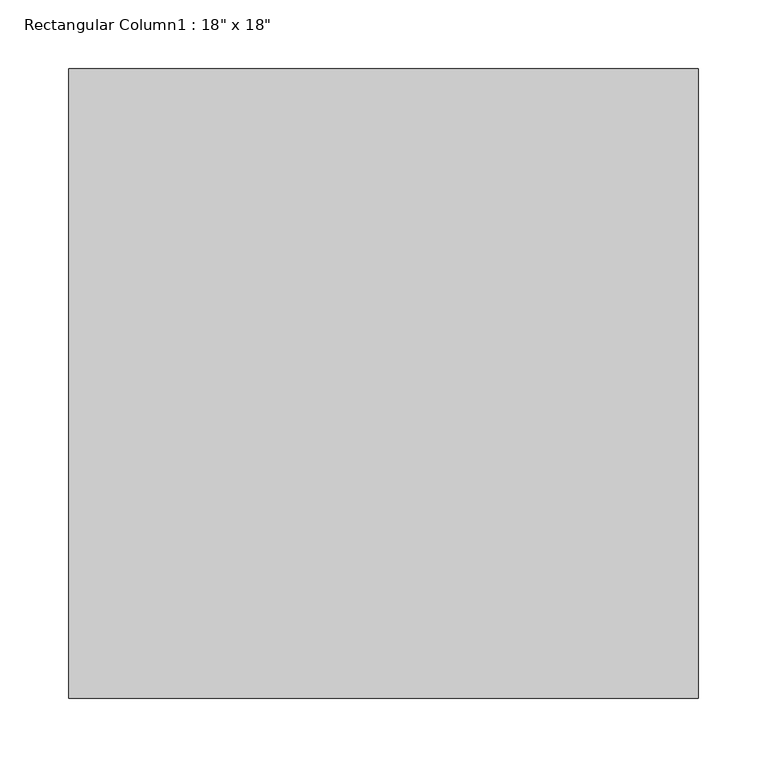
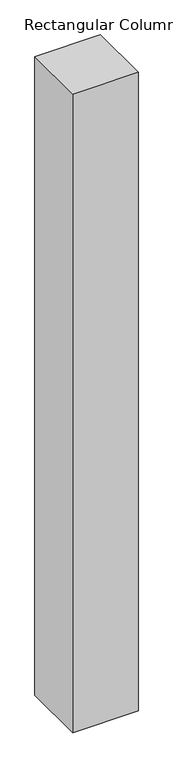
"""IFC4 building model written with IfcOpenShell, lengths in millimetres: column geometry."""

from ifc_helpers import new_model, si_unit, frame, origin, place, context, project, spatial, polyline, outline, extrude, source, transform, mapped, element, save


def column_773d994b(model_context):
    return source(origin(), model_context, "Body", "SweptSolid", [
        extrude(outline(polyline([(228.6, 228.6), (228.6, -228.6), (-228.6, -228.6), (-228.6, 228.6), (228.6, 228.6)])), frame((0.0, 0.0, 14935.2), z_axis=(0.0, 0.0, 1.0), x_axis=(1.0, 0.0, 0.0)), (0.0, 0.0, 1.0), 4724.4),
    ])


if __name__ == "__main__":
    model = new_model("IFC4")
    model_context = context("Model", 3, world=origin())
    ifc_project = project(units=[si_unit("LENGTHUNIT", "METRE", prefix="MILLI")], contexts=[model_context])
    site = spatial("IfcSite", under=ifc_project)
    building = spatial("IfcBuilding", under=site)
    placement = place(None, origin())
    column_shape = column_773d994b(model_context)
    element("IfcColumn", 1, ObjectType="Rectangular Column1 : 18\" x 18\"", at=placement, inside=building, context=model_context, shape_type="MappedRepresentation", body=[
        mapped(column_shape, transform((0.0, 0.0, 0.0), x_axis=(1.0, 0.0, 0.0), y_axis=(0.0, 1.0, 0.0), z_axis=(0.0, 0.0, 1.0))),
    ])
    save(model, "model.ifc")

# Revit data of these elements
# Type "Rectangular Column1 : 18\" x 18\""
#   Depth = 1' - 6"
#   Width = 1' - 6"
